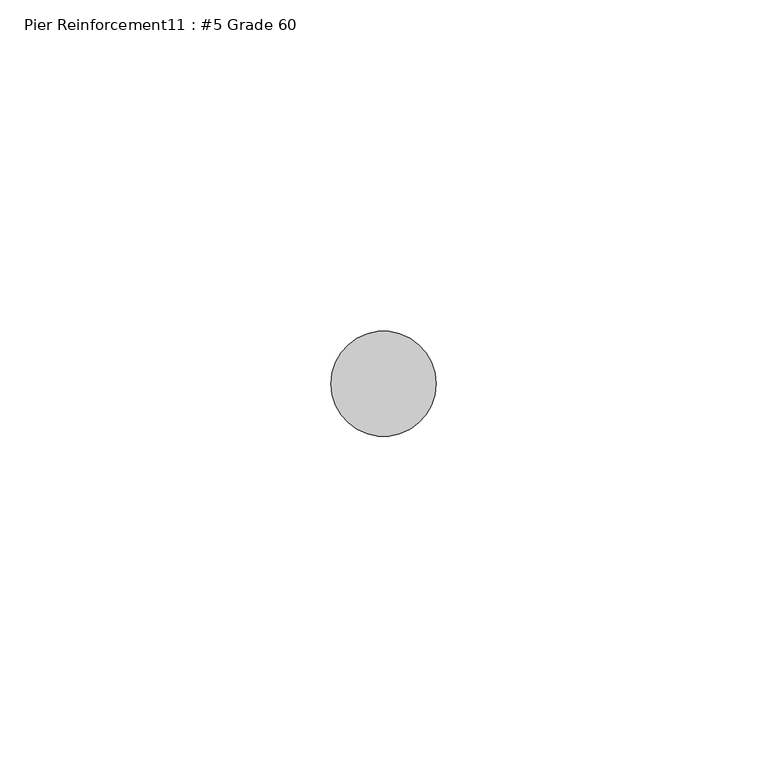
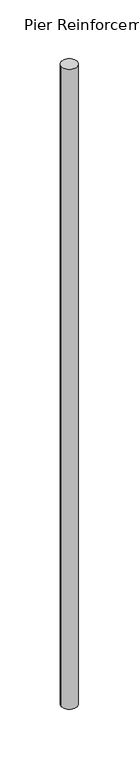
"""IFC4 building model written with IfcOpenShell, lengths in millimetres: proxy geometry, Pier Reinforcement11 : #5 Grade 60."""

from ifc_helpers import new_model, si_unit, point, frame, frame_2d, origin, place, context, project, spatial, circle_curve, trimmed, segment, composite_curve, outline, extrude, source, transform, mapped, element, save


def pier_reinforcement11_5_grade_60_3acffefc(model_context):
    return source(origin(), model_context, "Body", "SweptSolid", [
        extrude(outline(composite_curve([segment(trimmed(circle_curve(frame_2d((590226.0547365, -534096.6663841)), 7.9375), [point((590218.1172365, -534096.6663841))], [point((590233.9922365, -534096.6663841))], False, "CARTESIAN"), True, "CONTINUOUS"), segment(trimmed(circle_curve(frame_2d((590226.0547365, -534096.6663841)), 7.9375), [point((590233.9922365, -534096.6663841))], [point((590218.1172365, -534096.6663841))], False, "CARTESIAN"), True, "CONTINUOUS")], self_intersect=False)), frame((0.0, 0.0, -733.425), z_axis=(0.0, 0.0, 1.0), x_axis=(1.0, 0.0, 0.0)), (0.0, 0.0, 1.0), 685.8),
    ])


if __name__ == "__main__":
    model = new_model("IFC4")
    model_context = context("Model", 3, world=origin())
    ifc_project = project(units=[si_unit("LENGTHUNIT", "METRE", prefix="MILLI")], contexts=[model_context])
    site = spatial("IfcSite", under=ifc_project)
    building = spatial("IfcBuilding", under=site)
    placement = place(None, origin())
    pier_reinforcement11_5_grade_60_shape = pier_reinforcement11_5_grade_60_3acffefc(model_context)
    element("IfcBuildingElementProxy", 1, Name="Pier Reinforcement11 : #5 Grade 60", ObjectType="Pier Reinforcement11 : #5 Grade 60", at=placement, inside=building, context=model_context, shape_type="MappedRepresentation", body=[
        mapped(pier_reinforcement11_5_grade_60_shape, transform((0.0, 0.0, 0.0), x_axis=(1.0, 0.0, 0.0), y_axis=(0.0, 1.0, 0.0), z_axis=(0.0, 0.0, 1.0))),
    ])
    save(model, "model.ifc")

# Revit data of these elements
# Element 1 (IfcBuildingElementProxy, "Pier Reinforcement11 : #5 Grade 60")
#   Materials on its faces: "#4 GR. 60 REINF. @ 16\" O.C. EW."
# Materials
#   "#4 GR. 60 REINF. @ 16\" O.C. EW.": class "Generic", colour RGB 84 83 81, transparency 0, Cost = 0
